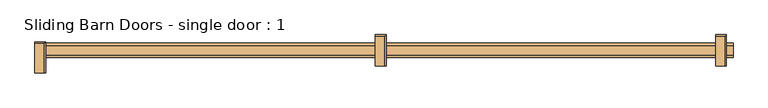
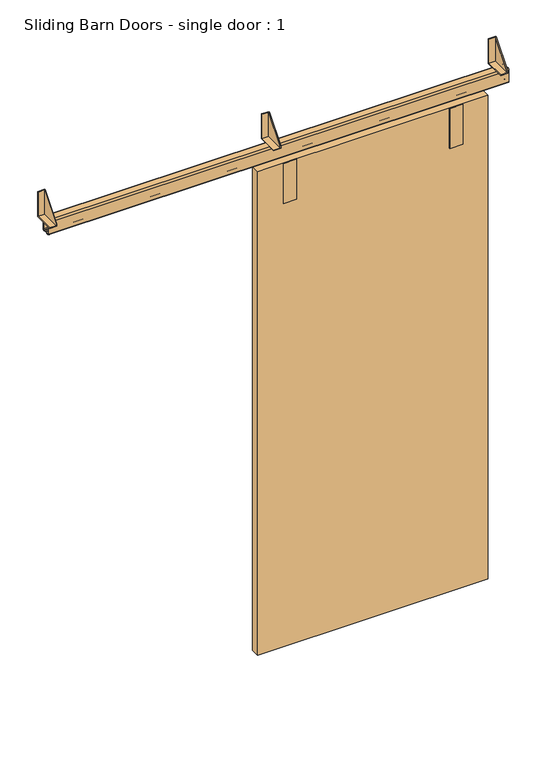
"""IFC4 building model written with IfcOpenShell, lengths in millimetres: door geometry, Sliding Barn Doors - single door : 1."""

from ifc_helpers import new_model, si_unit, point, frame, frame_2d, origin, place, context, project, spatial, polyline, circle_curve, trimmed, segment, composite_curve, outline, extrude, source, transform, mapped, element, save


def sliding_barn_doors_single_door_1_a8f467a9(model_context):
    return source(origin(), model_context, "Body", "SweptSolid", [
        extrude(outline(polyline([(-158.75, 2152.65), (-79.375, 2247.773), (-79.375, 2146.3), (-158.75, 2146.3), (-158.75, 2152.65)])), frame((-1385.9371094, 0.0, 0.0), z_axis=(1.0, 0.0, 0.0), x_axis=(0.0, 1.0, 0.0)), (0.0, 0.0, 1.0), 3.175),
        extrude(outline(polyline([(-76.2, 2143.125), (-158.75, 2143.125), (-158.75, 2146.3), (-79.375, 2146.3), (-79.375, 2247.773), (-76.2, 2247.773), (-76.2, 2143.125)])), frame((-1411.2378906, 0.0, 0.0), z_axis=(1.0, 0.0, 0.0), x_axis=(0.0, 1.0, 0.0)), (0.0, 0.0, 1.0), 28.4757812),
        extrude(outline(polyline([(-139.7, 2152.65), (-60.325, 2247.773), (-60.325, 2146.3), (-139.7, 2146.3), (-139.7, 2152.65)])), frame((-484.2371094, 0.0, 0.0), z_axis=(1.0, 0.0, 0.0), x_axis=(0.0, 1.0, 0.0)), (0.0, 0.0, 1.0), 3.175),
        extrude(outline(polyline([(-57.15, 2143.125), (-139.7, 2143.125), (-139.7, 2146.3), (-60.325, 2146.3), (-60.325, 2247.773), (-57.15, 2247.773), (-57.15, 2143.125)])), frame((-509.5378906, 0.0, 0.0), z_axis=(1.0, 0.0, 0.0), x_axis=(0.0, 1.0, 0.0)), (0.0, 0.0, 1.0), 28.4757813),
        extrude(outline(polyline([(-139.7, 2152.65), (-60.325, 2247.773), (-60.325, 2146.3), (-139.7, 2146.3), (-139.7, 2152.65)])), frame((417.4628906, 0.0, 0.0), z_axis=(1.0, 0.0, 0.0), x_axis=(0.0, 1.0, 0.0)), (0.0, 0.0, 1.0), 3.175),
        extrude(outline(polyline([(-57.15, 2143.125), (-139.7, 2143.125), (-139.7, 2146.3), (-60.325, 2146.3), (-60.325, 2247.773), (-57.15, 2247.773), (-57.15, 2143.125)])), frame((392.1621094, 0.0, 0.0), z_axis=(1.0, 0.0, 0.0), x_axis=(0.0, 1.0, 0.0)), (0.0, 0.0, 1.0), 28.4757813),
        extrude(outline(polyline([(-457.454, -117.475), (-457.454, -114.3), (-406.146, -114.3), (-406.146, -117.475), (-457.454, -117.475)])), frame((0.0, 0.0, 1889.252), z_axis=(0.0, 0.0, 1.0), x_axis=(1.0, 0.0, 0.0)), (0.0, 0.0, 1.0), 168.148),
        extrude(outline(polyline([(202.946, -117.475), (202.946, -114.3), (254.254, -114.3), (254.254, -117.475), (202.946, -117.475)])), frame((0.0, 0.0, 1889.252), z_axis=(0.0, 0.0, 1.0), x_axis=(1.0, 0.0, 0.0)), (0.0, 0.0, 1.0), 168.148),
        extrude(outline(polyline([(-558.8, -114.3), (-558.8, -79.375), (355.6, -79.375), (355.6, -114.3), (-558.8, -114.3)])), frame((0.0, 0.0, 25.4), z_axis=(0.0, 0.0, 1.0), x_axis=(1.0, 0.0, 0.0)), (0.0, 0.0, 1.0), 2032.0),
        extrude(outline(composite_curve([segment(trimmed(circle_curve(frame_2d((-85.725, 2136.775)), 6.35), [point((-85.725, 2143.125))], [point((-79.375, 2136.775))], False, "CARTESIAN"), True, "CONTINUOUS"), segment(polyline([(-79.375, 2136.775), (-79.375, 2088.515)]), True, "CONTINUOUS"), segment(trimmed(circle_curve(frame_2d((-85.725, 2088.515)), 6.35), [point((-79.375, 2088.515))], [point((-85.725, 2082.165))], False, "CARTESIAN"), True, "CONTINUOUS"), segment(polyline([(-85.725, 2082.165), (-91.1336853, 2082.165)]), True, "CONTINUOUS"), segment(trimmed(circle_curve(frame_2d((-91.1336853, 2083.7525)), 1.5875), [point((-91.1336853, 2082.165))], [point((-92.6920184, 2083.4495907))], False, "CARTESIAN"), True, "CONTINUOUS"), segment(polyline([(-92.6920184, 2083.4495907), (-94.1175341, 2090.7832331), (-92.6013971, 2090.7832331), (-91.2154749, 2083.6532812), (-85.725, 2083.6532812)]), True, "CONTINUOUS"), segment(trimmed(circle_curve(frame_2d((-85.725, 2088.515)), 4.8617187), [point((-85.725, 2083.6532812))], [point((-80.8632813, 2088.515))], True, "CARTESIAN"), True, "CONTINUOUS"), segment(polyline([(-80.8632813, 2088.515), (-80.8632813, 2136.775)]), True, "CONTINUOUS"), segment(trimmed(circle_curve(frame_2d((-85.725, 2136.775)), 4.8617187), [point((-80.8632813, 2136.775))], [point((-85.725, 2141.6367187))], True, "CARTESIAN"), True, "CONTINUOUS"), segment(polyline([(-85.725, 2141.6367187), (-111.252, 2141.6367187)]), True, "CONTINUOUS"), segment(trimmed(circle_curve(frame_2d((-111.252, 2136.775)), 4.8617187), [point((-111.252, 2141.6367187))], [point((-116.1137188, 2136.775))], True, "CARTESIAN"), True, "CONTINUOUS"), segment(polyline([(-116.1137188, 2136.775), (-116.1137188, 2088.515)]), True, "CONTINUOUS"), segment(trimmed(circle_curve(frame_2d((-111.252, 2088.515)), 4.8617187), [point((-116.1137188, 2088.515))], [point((-111.252, 2083.6532812))], True, "CARTESIAN"), True, "CONTINUOUS"), segment(polyline([(-111.252, 2083.6532812), (-105.7615251, 2083.6532812), (-104.3756029, 2090.7832331), (-102.8594659, 2090.7832331), (-104.2849816, 2083.4495907)]), True, "CONTINUOUS"), segment(trimmed(circle_curve(frame_2d((-105.8433147, 2083.7525)), 1.5875), [point((-104.2849816, 2083.4495907))], [point((-105.8433147, 2082.165))], False, "CARTESIAN"), True, "CONTINUOUS"), segment(polyline([(-105.8433147, 2082.165), (-111.252, 2082.165)]), True, "CONTINUOUS"), segment(trimmed(circle_curve(frame_2d((-111.252, 2088.515)), 6.35), [point((-111.252, 2082.165))], [point((-117.602, 2088.515))], False, "CARTESIAN"), True, "CONTINUOUS"), segment(polyline([(-117.602, 2088.515), (-117.602, 2136.775)]), True, "CONTINUOUS"), segment(trimmed(circle_curve(frame_2d((-111.252, 2136.775)), 6.35), [point((-117.602, 2136.775))], [point((-111.252, 2143.125))], False, "CARTESIAN"), True, "CONTINUOUS"), segment(polyline([(-111.252, 2143.125), (-85.725, 2143.125)]), True, "CONTINUOUS")], self_intersect=False)), frame((-1390.65, 0.0, 0.0), z_axis=(1.0, 0.0, 0.0), x_axis=(0.0, 1.0, 0.0)), (0.0, 0.0, 1.0), 1828.8),
    ])


if __name__ == "__main__":
    model = new_model("IFC4")
    model_context = context("Model", 3, world=origin())
    ifc_project = project(units=[si_unit("LENGTHUNIT", "METRE", prefix="MILLI")], contexts=[model_context])
    site = spatial("IfcSite", under=ifc_project)
    building = spatial("IfcBuilding", under=site)
    placement = place(None, origin())
    sliding_barn_doors_single_door_1_shape = sliding_barn_doors_single_door_1_a8f467a9(model_context)
    element("IfcDoor", 1, ObjectType="Sliding Barn Doors - single door : 1", at=placement, inside=building, context=model_context, shape_type="MappedRepresentation", body=[
        mapped(sliding_barn_doors_single_door_1_shape, transform((0.0, 0.0, 0.0), x_axis=(1.0, 0.0, 0.0), y_axis=(0.0, 1.0, 0.0), z_axis=(0.0, 0.0, 1.0))),
    ])
    save(model, "model.ifc")

# Revit data of these elements
# Type "Sliding Barn Doors - single door : 1"
#   Type Mark = "61"
#   OD_DS_Door_Material = "T.B.D."
#   OD_DS_Door_Type = "SLIDER"
#   OD_DS_Lockset = "-"
#   Analytic Construction = "<None>"
#   rail_overlap_left = 0' - 5 1/4"
#   rail_length = 6' - 0"
#   overlap_left = 0' - 2"
#   overlap = 0' - 0"
#   bracket_right = 3' - 7"
#   bracket_left = 0' - 4"
#   Thickness = 0' - 1 3/8"
#   Panel Width = 3' - 0"
#   Panel Height = 6' - 8"
#   Gap 2 = 0' - 0 1/2"
#   Gap 1 = 0' - 0 7/8"
#   Frame Projection Ext. = 0' - 1"
#   Frame Projection Int. = 0' - 1"
#   Frame Width = 0' - 3"
#   Height = 6' - 4"
#   Width = 2' - 0"
#   Bracket_offset = 0' - 5"
#   Door_4 = no
#   Door_3 = no
#   Hardware Material = Metal - Aluminum
#   Door Material = Closet_1
#   Function = (empty or 0)
#   Wall Closure = (empty or 0)
# Element 1 (IfcDoor, "Sliding Barn Doors - single door : 1")
#   Materials on its faces: "Metal - Aluminum", "Closet_1"
# Materials
#   "Metal - Aluminum": class "Metal", colour RGB 247 247 247, transparency 0
#   "Closet_1": class "Paint", colour RGB 200 194 183, transparency 0, Cost = 0
